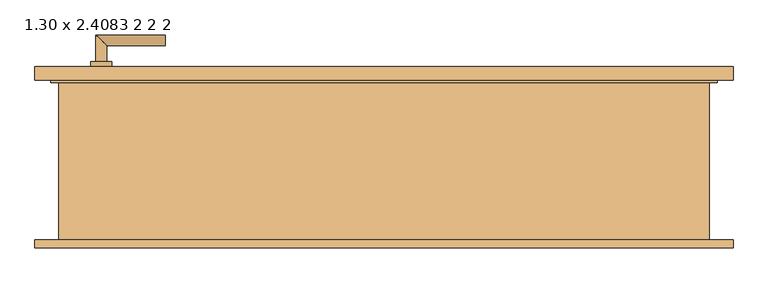
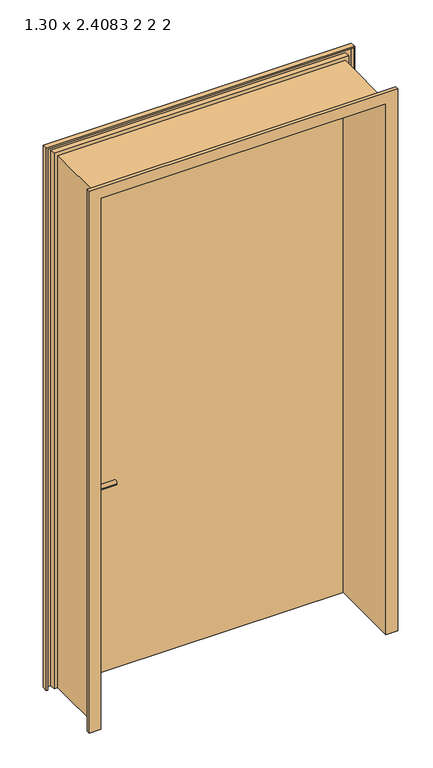
"""IFC4 building model written with IfcOpenShell, lengths in millimetres: door geometry, Drehflügel 1-flg - Stahlzarge : 1.30 x 2.4083 2 2 2."""

import ifcopenshell
import ifcopenshell.guid

model = None  # the IFC model being written
_history = None  # IfcOwnerHistory: only IFC2X3 demands one
_inside = {}  # id of a spatial element -> (the spatial element, [elements in it])
_under = {}  # id of a project, library or spatial element -> (it, [spatial elements below it])
_declared = {}  # id of a project -> (the project, [libraries it declares])
_typed = {}  # id of a type object -> (the type object, [elements of that type])
_made_of = {}  # id of a material, layer set ... -> (it, [elements and type objects made of it])


def new_model(schema):
    """Start an empty IFC model of exactly this schema.

    Asked for "IFC4X3", IfcOpenShell would pick the latest addendum, in which some entities
    have other attributes; the version numbers below select the first issue.
    IFC2X3 requires an IfcOwnerHistory on every rooted entity: one is made here for all.
    """
    global model, _history
    if schema == "IFC4X3":
        model = ifcopenshell.file(schema_version=(4, 3, 0, 0))
    else:
        model = ifcopenshell.file(schema=schema)
    _inside.clear()
    _under.clear()
    _declared.clear()
    _typed.clear()
    _made_of.clear()
    _history = None
    if model.schema == "IFC2X3":
        org = make("IfcOrganization", Name="unknown")
        user = make(
            "IfcPersonAndOrganization",
            ThePerson=make("IfcPerson", FamilyName="unknown"),
            TheOrganization=org,
        )
        app = make(
            "IfcApplication",
            ApplicationDeveloper=org,
            Version="unknown",
            ApplicationFullName="unknown",
            ApplicationIdentifier="unknown",
        )
        _history = make(
            "IfcOwnerHistory",
            OwningUser=user,
            OwningApplication=app,
            ChangeAction="ADDED",
            CreationDate=0,
        )
    return model


def make(cls, **values):
    """One entity of the class cls with the attributes given. An attribute that is None is left unset."""
    return model.create_entity(
        cls, **{name: value for name, value in values.items() if value is not None}
    )


def rooted(cls, **values):
    """An entity with a GlobalId (a new one), such as an element, a storey or a relation."""
    return make(cls, GlobalId=ifcopenshell.guid.new(), OwnerHistory=_history, **values)


def si_unit(unit_type, name, prefix=None):
    """IfcSIUnit, for example si_unit("LENGTHUNIT", "METRE", prefix="MILLI")."""
    return make("IfcSIUnit", UnitType=unit_type, Prefix=prefix, Name=name)


def assignment(units):
    """IfcUnitAssignment: the units of a project."""
    return None if units is None else make("IfcUnitAssignment", Units=units)


def point(xyz):
    """IfcCartesianPoint."""
    return None if xyz is None else make("IfcCartesianPoint", Coordinates=xyz)


def direction(xyz):
    """IfcDirection."""
    return None if xyz is None else make("IfcDirection", DirectionRatios=xyz)


def frame(location, z_axis=None, x_axis=None):
    """IfcAxis2Placement3D, a coordinate frame: its origin and axes. An axis left out is left unset."""
    return make(
        "IfcAxis2Placement3D",
        Location=point(location),
        Axis=direction(z_axis),
        RefDirection=direction(x_axis),
    )


def frame_2d(location, x_axis=None):
    """IfcAxis2Placement2D, a coordinate frame in the plane: its origin and x axis."""
    return make(
        "IfcAxis2Placement2D", Location=point(location), RefDirection=direction(x_axis)
    )


def origin():
    """The frame at (0, 0, 0) with its axes left unset."""
    return frame((0.0, 0.0, 0.0))


def place(relative_to, where):
    """IfcLocalPlacement: puts the frame where relative to a parent placement (None: the world)."""
    return make(
        "IfcLocalPlacement", PlacementRelTo=relative_to, RelativePlacement=where
    )


def context(
    kind, dimensions, precision=None, world=None, true_north=None, identifier=None
):
    """IfcGeometricRepresentationContext, for example the 3D "Model" context."""
    return make(
        "IfcGeometricRepresentationContext",
        ContextIdentifier=identifier,
        ContextType=kind,
        CoordinateSpaceDimension=dimensions,
        Precision=precision,
        WorldCoordinateSystem=world,
        TrueNorth=true_north,
    )


def project(units=None, contexts=None):
    """IfcProject with its units and contexts."""
    return rooted(
        "IfcProject",
        Name="project",
        RepresentationContexts=contexts,
        UnitsInContext=assignment(units),
    )


def spatial(cls, under=None, at=None, **own):
    """A site, building, storey or space (cls), placed at a placement, below another one or the project."""
    s = rooted(cls, ObjectPlacement=at, **own)
    if under is not None:
        _under.setdefault(under.id(), (under, []))[1].append(s)
    return s


def polyline(points):
    """IfcPolyline through the points."""
    return make("IfcPolyline", Points=[point(p) for p in points])


def circle_curve(where, radius):
    """IfcCircle in the frame where."""
    return make("IfcCircle", Position=where, Radius=radius)


def ellipse_curve(where, semi_axis1, semi_axis2):
    """IfcEllipse in the frame where."""
    return make(
        "IfcEllipse", Position=where, SemiAxis1=semi_axis1, SemiAxis2=semi_axis2
    )


def trimmed(basis, trim1, trim2, sense, master):
    """IfcTrimmedCurve: the piece of a basis curve between two trims."""
    return make(
        "IfcTrimmedCurve",
        BasisCurve=basis,
        Trim1=trim1,
        Trim2=trim2,
        SenseAgreement=sense,
        MasterRepresentation=master,
    )


def segment(curve, same_sense, transition):
    """IfcCompositeCurveSegment."""
    return make(
        "IfcCompositeCurveSegment",
        Transition=transition,
        SameSense=same_sense,
        ParentCurve=curve,
    )


def composite_curve(segments, self_intersect=None):
    """IfcCompositeCurve: segments joined end to end."""
    return make("IfcCompositeCurve", Segments=segments, SelfIntersect=self_intersect)


def outline(outer, holes=None, kind="AREA"):
    """IfcArbitraryClosedProfileDef: a profile drawn as a closed curve; with holes, ...WithVoids."""
    if holes is None:
        return make("IfcArbitraryClosedProfileDef", ProfileType=kind, OuterCurve=outer)
    return make(
        "IfcArbitraryProfileDefWithVoids",
        ProfileType=kind,
        OuterCurve=outer,
        InnerCurves=holes,
    )


def extrude(swept, where, along, depth):
    """IfcExtrudedAreaSolid: the profile swept, set in the frame where, extruded along a direction by depth."""
    return make(
        "IfcExtrudedAreaSolid",
        SweptArea=swept,
        Position=where,
        ExtrudedDirection=direction(along),
        Depth=depth,
    )


def faces_of(points, faces, orient=None, outer=None):
    """IfcFace entities. A face is a list of loops; a loop is a list of indices into points, from 0.

    orient and outer hold one flag for each loop. By default every Orientation is true, the
    first loop of a face is its IfcFaceOuterBound and the others are IfcFaceBound.
    """
    made = []
    for i, loops in enumerate(faces):
        bounds = []
        for j, loop in enumerate(loops):
            is_outer = j == 0 if outer is None else outer[i][j]
            bounds.append(
                make(
                    "IfcFaceOuterBound" if is_outer else "IfcFaceBound",
                    Bound=make("IfcPolyLoop", Polygon=[points[k] for k in loop]),
                    Orientation=True if orient is None else orient[i][j],
                )
            )
        made.append(make("IfcFace", Bounds=bounds))
    return made


def faceted_brep(points, faces, orient=None, outer=None, voids=None):
    """IfcFacetedBrep: a solid bounded by flat faces; with voids (closed shells), ...WithVoids."""
    shared = [point(p) for p in points]
    hull = make("IfcClosedShell", CfsFaces=faces_of(shared, faces, orient, outer))
    if voids is None:
        return make("IfcFacetedBrep", Outer=hull)
    return make(
        "IfcFacetedBrepWithVoids",
        Outer=hull,
        Voids=[
            make(cls, CfsFaces=faces_of(shared, fs, o, b)) for cls, fs, o, b in voids
        ],
    )


def shape(context_of_items, identifier, shape_type, items):
    """IfcShapeRepresentation: the items that make up one representation, for example the "Body"."""
    return make(
        "IfcShapeRepresentation",
        ContextOfItems=context_of_items,
        RepresentationIdentifier=identifier,
        RepresentationType=shape_type,
        Items=items,
    )


def source(mapping_origin, context_of_items, identifier, shape_type, items):
    """IfcRepresentationMap: a shape defined once, which mapped items show again and again."""
    return make(
        "IfcRepresentationMap",
        MappingOrigin=mapping_origin,
        MappedRepresentation=shape(context_of_items, identifier, shape_type, items),
    )


def transform(
    local_origin,
    x_axis=None,
    y_axis=None,
    z_axis=None,
    scale=None,
    scale2=None,
    scale3=None,
    uniform=True,
):
    """IfcCartesianTransformationOperator3D, or its non-uniform kind. x_axis, y_axis, z_axis: its Axis1, 2, 3."""
    if uniform:
        return make(
            "IfcCartesianTransformationOperator3D",
            Axis1=direction(x_axis),
            Axis2=direction(y_axis),
            LocalOrigin=point(local_origin),
            Scale=scale,
            Axis3=direction(z_axis),
        )
    return make(
        "IfcCartesianTransformationOperator3DnonUniform",
        Axis1=direction(x_axis),
        Axis2=direction(y_axis),
        LocalOrigin=point(local_origin),
        Scale=scale,
        Axis3=direction(z_axis),
        Scale2=scale2,
        Scale3=scale3,
    )


def mapped(mapping_source, mapping_target):
    """IfcMappedItem: shows the shape of a source again, moved by a transform."""
    return make(
        "IfcMappedItem", MappingSource=mapping_source, MappingTarget=mapping_target
    )


def made_of(thing, what):
    """Note that an element or type object is made of a material, layer set ...; save() writes the relation."""
    if what is not None:
        _made_of.setdefault(what.id(), (what, []))[1].append(thing)
    return thing


def element(
    cls,
    number,
    at=None,
    inside=None,
    cuts=None,
    type_object=None,
    material=None,
    context=None,
    identifier="Body",
    shape_type=None,
    held_by="IfcProductDefinitionShape",
    body=None,
    shapes=None,
    **own,
):
    """One element of the class cls, such as IfcWall. Its Tag is "e" and its number.

    at: its placement. inside: the storey or other place that contains it. cuts: it is an
    opening in that element (IfcRelVoidsElement). A single representation is given by context,
    identifier, shape_type and body (its items); several are given by shapes. held_by: the class
    of the entity that holds the representations. save() writes the other relations.
    """
    e = rooted(cls, Tag="e%d" % number, ObjectPlacement=at, **own)
    if body is not None:
        shapes = [shape(context, identifier, shape_type, body)]
    if shapes is not None:
        e.Representation = make(held_by, Representations=shapes)
    if inside is not None:
        _inside.setdefault(inside.id(), (inside, []))[1].append(e)
    if cuts is not None:
        rooted(
            "IfcRelVoidsElement", RelatingBuildingElement=cuts, RelatedOpeningElement=e
        )
    if type_object is not None:
        _typed.setdefault(type_object.id(), (type_object, []))[1].append(e)
    return made_of(e, material)


def aggregate(whole, parts):
    """IfcRelAggregates: a whole, such as a stair, and the parts it consists of."""
    return rooted("IfcRelAggregates", RelatingObject=whole, RelatedObjects=parts)


def save(model, path):
    """Write the relations noted so far, then the file.

    IfcRelAggregates (storeys below a building ...), IfcRelContainedInSpatialStructure (elements
    in a storey), IfcRelDefinesByType, IfcRelAssociatesMaterial and IfcRelDeclares: one each for
    every whole, place, type object, material and project.
    """
    for whole, parts in _under.values():
        aggregate(whole, parts)
    for where, things in _inside.values():
        rooted(
            "IfcRelContainedInSpatialStructure",
            RelatedElements=things,
            RelatingStructure=where,
        )
    for kind, things in _typed.values():
        rooted("IfcRelDefinesByType", RelatedObjects=things, RelatingType=kind)
    for what, things in _made_of.values():
        rooted("IfcRelAssociatesMaterial", RelatedObjects=things, RelatingMaterial=what)
    for by, libraries in _declared.values():
        rooted("IfcRelDeclares", RelatingContext=by, RelatedDefinitions=libraries)
    model.write(path)


def plane_surface(at):
    """IfcPlane: the flat surface through the origin of the frame at, square to its z axis."""
    return make("IfcPlane", Position=at)


def cylinder_surface(at, radius):
    """IfcCylindricalSurface: all points at the distance radius from the z axis of the frame at."""
    return make("IfcCylindricalSurface", Position=at, Radius=radius)


def advanced_brep(points, edges, surfaces, faces):
    """IfcAdvancedBrep: a solid bounded by faces that lie on surfaces and meet in shared edges.

    An edge is (start, end): straight between two places in points (the first is 0);
    or (start, end, curve); or (start, end, curve, False) where it runs against its curve.
    A face is (place in surfaces, loops), or (place, loops, False) where it looks against
    its surface's normal. A loop lists edges by number (the first is 1), with a minus sign
    where the edge is run from its end to its start. The first loop is the outer one.
    """
    corners = [point(p) for p in points]
    vertices = [make("IfcVertexPoint", VertexGeometry=c) for c in corners]
    made = []
    for start, end, *more in edges:
        made.append(
            make(
                "IfcEdgeCurve",
                EdgeStart=vertices[start],
                EdgeEnd=vertices[end],
                EdgeGeometry=more[0] if more else make("IfcPolyline", Points=[corners[start], corners[end]]),
                SameSense=more[1] if len(more) > 1 else True,
            )
        )
    hull = []
    for where, loops, *sense in faces:
        bounds = []
        for j, loop in enumerate(loops):
            ring = [make("IfcOrientedEdge", EdgeElement=made[abs(k) - 1], Orientation=k > 0) for k in loop]
            bounds.append(
                make(
                    "IfcFaceOuterBound" if j == 0 else "IfcFaceBound",
                    Bound=make("IfcEdgeLoop", EdgeList=ring),
                    Orientation=True,
                )
            )
        hull.append(make("IfcAdvancedFace", Bounds=bounds, FaceSurface=surfaces[where], SameSense=sense[0] if sense else True))
    return make("IfcAdvancedBrep", Outer=make("IfcClosedShell", CfsFaces=hull))


def door_1_30_x_2_4083_2_2_2_ebc270b9(model_context):
    return source(origin(), model_context, "Body", "SolidModel", [
        advanced_brep(
        [(-540.0, 139.4346141, 915.0), (-520.0, 139.4346141, 915.0), (-540.0, 69.4346141, 915.0), (-520.0, 89.4346141, 915.0), (-410.0, 69.4346141, 915.0), (-410.0, 89.4346141, 915.0)],
        [
            (0, 1, circle_curve(frame((-530.0, 139.4346141, 915.0), z_axis=(0.0, 1.0, 0.0), x_axis=(1.0, 0.0, 0.0)), 10.0)),
            (1, 0, circle_curve(frame((-530.0, 139.4346141, 915.0), z_axis=(0.0, 1.0, 0.0), x_axis=(1.0, 0.0, 0.0)), 10.0)),
            (0, 2),
            (2, 3, ellipse_curve(frame((-530.0, 79.4346141, 915.0), z_axis=(-0.7071067811865385, 0.7071067811865565, 0.0), x_axis=(0.7071067811865563, 0.7071067811865386, 0.0)), 14.1421356, 10.0)),
            (3, 1),
            (3, 2, ellipse_curve(frame((-530.0, 79.4346141, 915.0), z_axis=(-0.7071067811865385, 0.7071067811865565, 0.0), x_axis=(0.7071067811865563, 0.7071067811865386, 0.0)), 14.1421356, 10.0)),
            (4, 5, circle_curve(frame((-410.0, 79.4346141, 915.0), z_axis=(1.0, 0.0, 0.0), x_axis=(0.0, 1.0, 0.0)), 10.0)),
            (5, 4, circle_curve(frame((-410.0, 79.4346141, 915.0), z_axis=(1.0, 0.0, 0.0), x_axis=(0.0, 1.0, 0.0)), 10.0)),
            (2, 4),
            (5, 3),
        ],
        [
            plane_surface(frame((-530.0, 139.4346141, -372.7526403), z_axis=(0.0, 1.0, 0.0), x_axis=(0.0, 0.0, 1.0))),
            cylinder_surface(frame((-530.0, 139.4346141, 915.0), z_axis=(0.0, 1.0, 0.0), x_axis=(1.0, 0.0, 0.0)), 10.0),
            plane_surface(frame((-410.0, 79.4346141, -372.7526403), z_axis=(1.0, 0.0, 0.0), x_axis=(0.0, 0.0, 1.0))),
            cylinder_surface(frame((-530.0, 79.4346141, 915.0), z_axis=(-1.0, 0.0, 0.0), x_axis=(0.0, 1.0, 0.0)), 10.0),
        ],
        [
            (0, [[1, 2]]),
            (1, [[-1, 3, 4, 5]]),
            (1, [[-2, -5, 6, -3]]),
            (2, [[7, 8]]),
            (3, [[-4, 9, -8, 10]]),
            (3, [[-6, -10, -7, -9]]),
        ],
    ),
        advanced_brep(
        [(-520.0, 199.4346141, 915.0), (-540.0, 199.4346141, 915.0), (-520.0, 229.4346141, 915.0), (-540.0, 249.4346141, 915.0), (-410.0, 229.4346141, 915.0), (-410.0, 249.4346141, 915.0)],
        [
            (0, 1, circle_curve(frame((-530.0, 199.4346141, 915.0), z_axis=(0.0, -1.0, 0.0), x_axis=(-1.0, 0.0, 0.0)), 10.0)),
            (1, 0, circle_curve(frame((-530.0, 199.4346141, 915.0), z_axis=(0.0, -1.0, 0.0), x_axis=(-1.0, 0.0, 0.0)), 10.0)),
            (0, 2),
            (2, 3, ellipse_curve(frame((-530.0, 239.4346141, 915.0), z_axis=(-0.7071067811865475, -0.7071067811865475, 0.0), x_axis=(0.7071067811865474, -0.7071067811865476, 0.0)), 14.1421356, 10.0)),
            (3, 1),
            (3, 2, ellipse_curve(frame((-530.0, 239.4346141, 915.0), z_axis=(-0.7071067811865475, -0.7071067811865475, 0.0), x_axis=(0.7071067811865474, -0.7071067811865476, 0.0)), 14.1421356, 10.0)),
            (4, 5, circle_curve(frame((-410.0, 239.4346141, 915.0), z_axis=(1.0, 0.0, 0.0), x_axis=(0.0, 1.0, 0.0)), 10.0)),
            (5, 4, circle_curve(frame((-410.0, 239.4346141, 915.0), z_axis=(1.0, 0.0, 0.0), x_axis=(0.0, 1.0, 0.0)), 10.0)),
            (2, 4),
            (5, 3),
        ],
        [
            plane_surface(frame((-530.0, 199.4346141, -372.7526403), z_axis=(0.0, -1.0, 0.0), x_axis=(0.0, 0.0, 1.0))),
            cylinder_surface(frame((-530.0, 199.4346141, 915.0), z_axis=(0.0, -1.0, 0.0), x_axis=(-1.0, 0.0, 0.0)), 10.0),
            plane_surface(frame((-410.0, 239.4346141, -372.7526403), z_axis=(1.0, 0.0, 0.0), x_axis=(0.0, 0.0, 1.0))),
            cylinder_surface(frame((-530.0, 239.4346141, 915.0), z_axis=(-1.0, 0.0, 0.0), x_axis=(0.0, 1.0, 0.0)), 10.0),
        ],
        [
            (0, [[1, 2]]),
            (1, [[-1, 3, 4, 5]]),
            (1, [[-2, -5, 6, -3]]),
            (2, [[7, 8]]),
            (3, [[-4, 9, -8, 10]]),
            (3, [[-6, -10, -7, -9]]),
        ],
    ),
        extrude(outline(composite_curve([segment(trimmed(circle_curve(frame_2d((915.0, -530.0)), 20.0), [point((915.0, -550.0))], [point((915.0, -510.0))], False, "CARTESIAN"), True, "CONTINUOUS"), segment(trimmed(circle_curve(frame_2d((915.0, -530.0)), 20.0), [point((915.0, -510.0))], [point((915.0, -550.0))], False, "CARTESIAN"), True, "CONTINUOUS")], self_intersect=False)), frame((0.0, 129.4346141, 0.0), z_axis=(0.0, 1.0, 0.0), x_axis=(0.0, 0.0, 1.0)), (0.0, 0.0, 1.0), 10.0),
        extrude(outline(composite_curve([segment(trimmed(circle_curve(frame_2d((915.0, -530.0)), 20.0), [point((915.0, -550.0))], [point((915.0, -510.0))], False, "CARTESIAN"), True, "CONTINUOUS"), segment(trimmed(circle_curve(frame_2d((915.0, -530.0)), 20.0), [point((915.0, -510.0))], [point((915.0, -550.0))], False, "CARTESIAN"), True, "CONTINUOUS")], self_intersect=False)), frame((0.0, 189.4346141, 0.0), z_axis=(0.0, 1.0, 0.0), x_axis=(0.0, 0.0, 1.0)), (0.0, 0.0, 1.0), 10.0),
        extrude(outline(polyline([(620.0, 164.4346141), (-620.0, 164.4346141), (-620.0, 189.4346141), (620.0, 189.4346141), (620.0, 164.4346141)])), frame((0.0, 0.0, 15.0), z_axis=(0.0, 0.0, 1.0), x_axis=(1.0, 0.0, 0.0)), (0.0, 0.0, 1.0), 2398.3),
        faceted_brep([(654.4603207, -150.5653859, 15.0), (605.0, -150.5653859, 15.0), (605.0, 164.4346141, 15.0), (620.0, 164.4346141, 15.0), (620.0, 189.4346141, 15.0), (654.4603207, 189.4346141, 15.0), (654.4603207, 164.4346141, 15.0), (649.4603207, 164.4346141, 15.0), (649.4603207, 184.4346141, 15.0), (625.0, 184.4346141, 15.0), (625.0, 159.4346141, 15.0), (610.0, 159.4346141, 15.0), (610.0, -145.5653859, 15.0), (649.4603207, -145.5653859, 15.0), (649.4603207, -135.5653859, 15.0), (654.4603207, -135.5653859, 15.0), (654.4603207, -150.5653859, 2447.7603207), (-654.4603207, -150.5653859, 2447.7603207), (-654.4603207, -150.5653859, 15.0), (-605.0, -150.5653859, 15.0), (-605.0, -150.5653859, 2398.3), (605.0, -150.5653859, 2398.3), (605.0, 164.4346141, 2398.3), (-605.0, 164.4346141, 2398.3), (-605.0, 164.4346141, 15.0), (-620.0, 164.4346141, 15.0), (-620.0, 164.4346141, 2413.3), (620.0, 164.4346141, 2413.3), (620.0, 189.4346141, 2413.3), (-620.0, 189.4346141, 2413.3), (-620.0, 189.4346141, 15.0), (-654.4603207, 189.4346141, 15.0), (-654.4603207, 189.4346141, 2447.7603207), (654.4603207, 189.4346141, 2447.7603207), (654.4603207, 164.4346141, 2447.7603207), (-654.4603207, 164.4346141, 2447.7603207), (-654.4603207, 164.4346141, 15.0), (-649.4603207, 164.4346141, 15.0), (-649.4603207, 164.4346141, 2442.7603207), (649.4603207, 164.4346141, 2442.7603207), (649.4603207, 184.4346141, 2442.7603207), (-649.4603207, 184.4346141, 2442.7603207), (-649.4603207, 184.4346141, 15.0), (-625.0, 184.4346141, 15.0), (-625.0, 184.4346141, 2418.3), (625.0, 184.4346141, 2418.3), (625.0, 159.4346141, 2418.3), (-625.0, 159.4346141, 2418.3), (-625.0, 159.4346141, 15.0), (-610.0, 159.4346141, 15.0), (-610.0, 159.4346141, 2403.3), (610.0, 159.4346141, 2403.3), (610.0, -145.5653859, 2403.3), (-610.0, -145.5653859, 2403.3), (-610.0, -145.5653859, 15.0), (-649.4603207, -145.5653859, 15.0), (-649.4603207, -145.5653859, 2442.7603207), (649.4603207, -145.5653859, 2442.7603207), (649.4603207, -135.5653859, 2442.7603207), (-649.4603207, -135.5653859, 2442.7603207), (-649.4603207, -135.5653859, 15.0), (-654.4603207, -135.5653859, 15.0), (-654.4603207, -135.5653859, 2447.7603207), (654.4603207, -135.5653859, 2447.7603207)], [[[0, 1, 2, 3, 4, 5, 6, 7, 8, 9, 10, 11, 12, 13, 14, 15]], [[1, 0, 16, 17, 18, 19, 20, 21]], [[2, 1, 21, 22]], [[3, 2, 22, 23, 24, 25, 26, 27]], [[4, 3, 27, 28]], [[5, 4, 28, 29, 30, 31, 32, 33]], [[6, 5, 33, 34]], [[7, 6, 34, 35, 36, 37, 38, 39]], [[8, 7, 39, 40]], [[9, 8, 40, 41, 42, 43, 44, 45]], [[10, 9, 45, 46]], [[11, 10, 46, 47, 48, 49, 50, 51]], [[12, 11, 51, 52]], [[13, 12, 52, 53, 54, 55, 56, 57]], [[14, 13, 57, 58]], [[15, 14, 58, 59, 60, 61, 62, 63]], [[0, 15, 63, 16]], [[17, 62, 61, 18]], [[18, 61, 60, 55, 54, 49, 48, 43, 42, 37, 36, 31, 30, 25, 24, 19]], [[23, 20, 19, 24]], [[29, 26, 25, 30]], [[35, 32, 31, 36]], [[41, 38, 37, 42]], [[47, 44, 43, 48]], [[53, 50, 49, 54]], [[59, 56, 55, 60]], [[22, 21, 20, 23]], [[28, 27, 26, 29]], [[34, 33, 32, 35]], [[40, 39, 38, 41]], [[46, 45, 44, 47]], [[52, 51, 50, 53]], [[58, 57, 56, 59]], [[16, 63, 62, 17]]]),
    ])


if __name__ == "__main__":
    model = new_model("IFC4")
    model_context = context("Model", 3, world=origin())
    ifc_project = project(units=[si_unit("LENGTHUNIT", "METRE", prefix="MILLI")], contexts=[model_context])
    site = spatial("IfcSite", under=ifc_project)
    building = spatial("IfcBuilding", under=site)
    placement = place(None, origin())
    door_1_30_x_2_4083_2_2_2_shape = door_1_30_x_2_4083_2_2_2_ebc270b9(model_context)
    element("IfcDoor", 1, ObjectType="Drehflügel 1-flg - Stahlzarge : 1.30 x 2.4083 2 2 2", at=placement, inside=building, context=model_context, shape_type="MappedRepresentation", body=[
        mapped(door_1_30_x_2_4083_2_2_2_shape, transform((0.0, 0.0, 0.0), x_axis=(1.0, 0.0, 0.0), y_axis=(0.0, 1.0, 0.0), z_axis=(0.0, 0.0, 1.0))),
    ])
    save(model, "model.ifc")

# Revit data of these elements
# Type "Drehflügel 1-flg - Stahlzarge : 1.30 x 2.4083 2 2 2"
#   Type Mark = "26"
#   Operation = "SingleSwingRight"
#   Keynote = "16.03"
#   Analytic Construction = "Metall"
#   Thermal Resistance (R) = 0.270117 (m²·K)/W
#   Heat Transfer Coefficient (U) = 3.7021 W/(m²·K)
#   Rough Width = 1.260 m
#   Rough Height [instance default] = 2.5083 m
#   Höhe Türgriff [instance default] = 0.900 m
#   Height = 2.4083 m
#   Fußbodenaufbau [instance default] = 0.100 m
#   Width = 1.260 m
#   Sichtbarkeit Sturzlinien [instance default] = yes
#   Türgriff auswählen [instance default] = element 221079
#   Türgriff [instance default] = none
#   Türflügel [instance default] = none
#   Rahmen/Pfosten [instance default] = Metall - Lackiert - Grau
#   Visual Light Transmittance = 0
#   Solar Heat Gain Coefficient = 0
#   Function = (empty or 0)
#   Wall Closure = (empty or 0)
# Element 1 (IfcDoor, "Drehflügel 1-flg - Stahlzarge : 1.30 x 2.4083 2 2 2")
#   Rough Height = 2.4233 m
#   Fußbodenaufbau = 0.015 m
#   Materials on its faces: "Metall - Lackiert - Grau", "Metall - Chrom", "Holz - Birke"
# Materials
#   "Metall - Lackiert - Grau": class "Farbe 1", colour RGB 98 98 98, transparency 0, Cost = 0
#   "Metall - Chrom": class "Metall", colour RGB 247 247 247, transparency 0, Cost = 0
#   "Holz - Birke": class "Holz", colour RGB 213 164 103, transparency 0, Cost = 0
